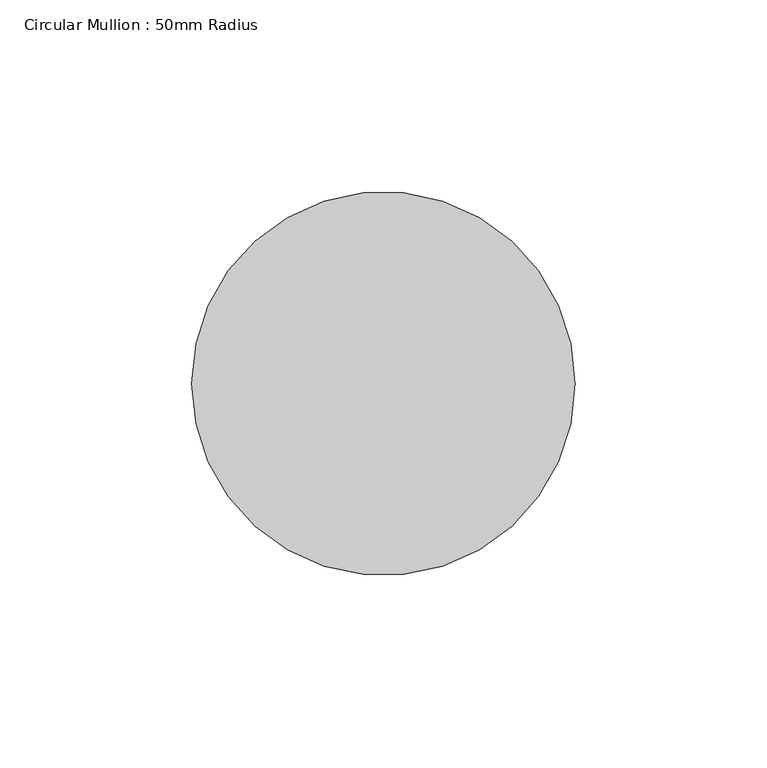
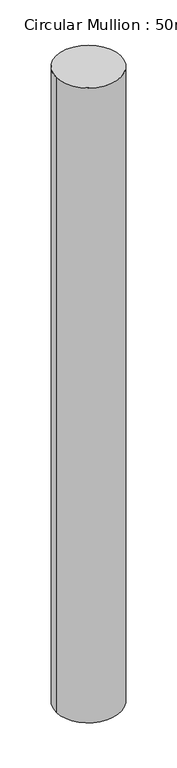
"""IFC4 building model written with IfcOpenShell, lengths in millimetres: member geometry, Circular Mullion : 50mm Radius."""

from ifc_helpers import new_model, si_unit, point, frame, origin, origin_2d, place, context, project, spatial, circle_curve, trimmed, segment, composite_curve, outline, extrude, source, transform, mapped, element, save


def circular_mullion_50mm_radius_9408c18b(model_context):
    return source(origin(), model_context, "Body", "SweptSolid", [
        extrude(outline(composite_curve([segment(trimmed(circle_curve(origin_2d(), 50.0), [point((50.0, 0.0))], [point((-50.0, 0.0))], False, "CARTESIAN"), True, "CONTINUOUS"), segment(trimmed(circle_curve(origin_2d(), 50.0), [point((-50.0, 0.0))], [point((50.0, 0.0))], False, "CARTESIAN"), True, "CONTINUOUS")], self_intersect=False)), frame((0.0, 0.0, -1037.4408285), z_axis=(0.0, 0.0, 1.0), x_axis=(1.0, 0.0, 0.0)), (0.0, 0.0, 1.0), 1037.4408285),
    ])


if __name__ == "__main__":
    model = new_model("IFC4")
    model_context = context("Model", 3, world=origin())
    ifc_project = project(units=[si_unit("LENGTHUNIT", "METRE", prefix="MILLI")], contexts=[model_context])
    site = spatial("IfcSite", under=ifc_project)
    building = spatial("IfcBuilding", under=site)
    placement = place(None, origin())
    circular_mullion_50mm_radius_shape = circular_mullion_50mm_radius_9408c18b(model_context)
    element("IfcMember", 1, ObjectType="Circular Mullion : 50mm Radius", at=placement, inside=building, context=model_context, shape_type="MappedRepresentation", body=[
        mapped(circular_mullion_50mm_radius_shape, transform((0.0, 0.0, 0.0), x_axis=(1.0, 0.0, 0.0), y_axis=(0.0, 1.0, 0.0), z_axis=(0.0, 0.0, 1.0))),
    ])
    save(model, "model.ifc")

# Revit data of these elements
# Type "Circular Mullion : 50mm Radius"
#   built-in parameter 1007350 = 0.164042 (stored number, unit not read)
# Element 1 (IfcMember, "Circular Mullion : 50mm Radius")
#   Materials on its faces: "Aluminium"
# Materials
#   "Aluminium": class "Metal", colour RGB 247 247 247, transparency 0, Description = "Aluminium 6061", Cost = 0
